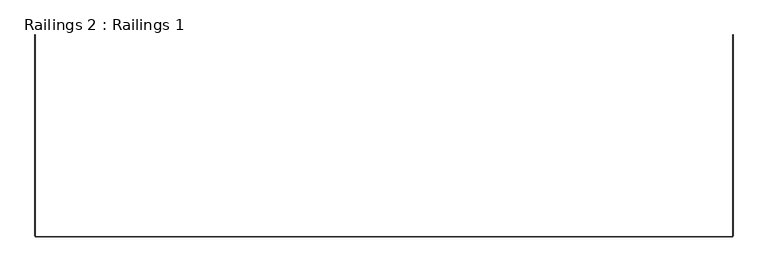
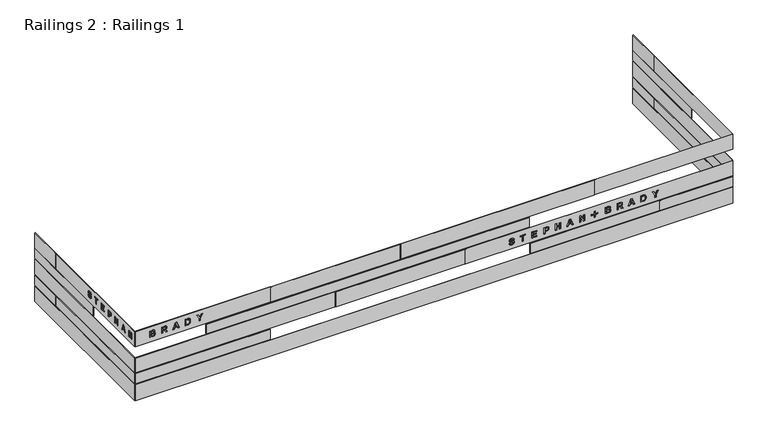
"""IFC4 building model written with IfcOpenShell, lengths in millimetres: railing geometry, Railings 2 : Railings 1."""

from ifc_helpers import new_model, si_unit, frame, origin, place, context, project, spatial, polyline, outline, extrude, source, transform, mapped, element, save


def railings_2_railings_1_346be623(model_context):
    return source(origin(), model_context, "Body", "SweptSolid", [
        extrude(outline(polyline([(-635.7738191, 4458.9611535), (-635.7738191, 4170.7510115), (-3091.5141621, 4170.7510115), (-3091.5141621, 4458.9611535), (-635.7738191, 4458.9611535)]), holes=[polyline([(-1665.1455091, 4296.7227585), (-1666.4698877, 4291.2327602), (-1668.3360732, 4286.5234788), (-1670.7440658, 4282.5949142), (-1673.6938655, 4279.4470663), (-1677.1955571, 4277.0342631), (-1681.2592258, 4275.3108322), (-1685.8848714, 4274.2767736), (-1691.072494, 4273.9320875), (-1696.5086477, 4274.2386941), (-1701.2307383, 4275.1585142), (-1705.2387656, 4276.6915475), (-1708.5327298, 4278.8377942), (-1711.7959882, 4282.2929121), (-1713.7539433, 4286.1173232), (-1714.406595, 4290.3110276), (-1713.7892085, 4294.2128728), (-1711.9370492, 4297.4868988), (-1708.5464083, 4300.2541255), (-1703.3135771, 4302.6355726), (-1701.1988373, 4303.3094256), (-1698.2227703, 4304.1647435), (-1694.3853762, 4305.2015261), (-1689.686655, 4306.4197736), (-1684.1266067, 4307.8194858), (-1678.0225, 4309.4734745), (-1672.5571346, 4311.2490498), (-1667.7305106, 4313.1462116), (-1663.5426279, 4315.1649599), (-1659.9934866, 4317.3052948), (-1657.0830867, 4319.5672161), (-1653.7434245, 4322.9544825), (-1651.0109737, 4326.5802851), (-1648.8857341, 4330.444624), (-1647.3677059, 4334.5474991), (-1646.4568889, 4338.8889105), (-1646.1532833, 4343.4688582), (-1646.4744958, 4347.9329702), (-1647.4381333, 4352.2502124), (-1649.0441959, 4356.4205848), (-1651.2926834, 4360.4440874), (-1654.1456904, 4364.1586649), (-1657.5653112, 4367.4022621), (-1661.5515457, 4370.174879), (-1666.104394, 4372.4765156), (-1670.133565, 4373.9641411), (-1674.4832299, 4375.1211831), (-1679.1533885, 4375.9476417), (-1684.144041, 4376.4435168), (-1689.4551873, 4376.6088085), (-1695.612066, 4376.4087649), (-1701.318061, 4375.8086338), (-1706.5731724, 4374.8084155), (-1711.3774, 4373.4081098), (-1715.730744, 4371.6077167), (-1719.6332044, 4369.4072363), (-1723.084781, 4366.8066685), (-1726.5506664, 4363.3570633), (-1729.4206749, 4359.5430077), (-1731.6948064, 4355.3645016), (-1733.373061, 4350.8215451), (-1734.4554386, 4345.9141382), (-1734.9419392, 4340.6422808), (-1710.964254, 4339.5739681), (-1709.5483894, 4345.1168707), (-1707.3508677, 4349.514387), (-1704.3716889, 4352.7665172), (-1701.5281294, 4354.5248978), (-1698.0524616, 4355.7808839), (-1693.9446857, 4356.5344756), (-1689.2048015, 4356.7856728), (-1684.2705786, 4356.5168558), (-1679.9025057, 4355.7104049), (-1676.100583, 4354.3663201), (-1672.8648103, 4352.4846013), (-1670.0131944, 4349.2597251), (-1669.0626557, 4345.1010026), (-1669.95338, 4341.1857107), (-1672.6255528, 4337.8787636), (-1674.9577759, 4336.3407271), (-1678.3266332, 4334.7772441), (-1682.7321248, 4333.1883144), (-1688.1742507, 4331.5739381), (-1694.6530108, 4329.9341152), (-1700.230818, 4328.5491881), (-1705.302444, 4327.1486505), (-1709.8678888, 4325.7325025), (-1713.9271525, 4324.300744), (-1717.4802351, 4322.8533751), (-1720.5271365, 4321.3903956), (-1724.4901292, 4318.9818814), (-1727.9976748, 4316.1686927), (-1731.0497732, 4312.9508296), (-1733.6464246, 4309.328292), (-1735.7192364, 4305.2782439), (-1737.1998162, 4300.7778491), (-1738.0881642, 4295.8271077), (-1738.3842801, 4290.4260196), (-1738.0300886, 4285.4065379), (-1736.9675139, 4280.5489956), (-1735.196556, 4275.8533927), (-1732.7172151, 4271.319729), (-1729.5901748, 4267.1529501), (-1725.8761189, 4263.5580014), (-1721.5750474, 4260.5348828), (-1716.6869604, 4258.0835943), (-1712.3377036, 4256.5245254), (-1707.5804848, 4255.3119163), (-1702.4153042, 4254.445767), (-1696.8421616, 4253.9260774), (-1690.8610571, 4253.7528475), (-1685.3975175, 4253.9153664), (-1680.2603487, 4254.4029232), (-1675.4495509, 4255.2155178), (-1670.965124, 4256.3531503), (-1666.8070681, 4257.8158206), (-1662.975383, 4259.6035288), (-1659.4700689, 4261.7162748), (-1656.2911257, 4264.1540587), (-1653.0428101, 4267.3199343), (-1650.1910238, 4270.8740121), (-1647.7357669, 4274.8162919), (-1645.6770393, 4279.1467737), (-1644.014841, 4283.8654576), (-1642.7491721, 4288.9723436), (-1641.8800324, 4294.4674317), (-1665.1455091, 4296.7227585)]), polyline([(-1876.840094, 4354.6490474), (-1841.5857748, 4354.6490474), (-1841.5857748, 4374.709586), (-1935.9533971, 4374.709586), (-1935.9533971, 4354.6490474), (-1900.8177792, 4354.6490474), (-1900.8177792, 4256.0081743), (-1876.840094, 4256.0081743), (-1876.840094, 4354.6490474)]), polyline([(-2055.9253864, 4374.709586), (-2143.7644311, 4374.709586), (-2143.7644311, 4354.6490474), (-2079.9030716, 4354.6490474), (-2079.9030716, 4328.297334), (-2139.3724788, 4328.297334), (-2139.3724788, 4308.2367954), (-2079.9030716, 4308.2367954), (-2079.9030716, 4276.0687129), (-2146.0197579, 4276.0687129), (-2146.0197579, 4256.0081743), (-2055.9253864, 4256.0081743), (-2055.9253864, 4374.709586)]), polyline([(-2276.947415, 4374.709586), (-2315.3565952, 4374.709586), (-2322.2116017, 4374.6600755), (-2328.2220971, 4374.5115442), (-2333.3880815, 4374.263992), (-2337.7095548, 4373.9174189), (-2341.1865169, 4373.4718249), (-2343.818968, 4372.9272101), (-2348.70578, 4371.1985628), (-2353.1782961, 4368.6852575), (-2357.2365166, 4365.3872941), (-2360.8804412, 4361.3046726), (-2363.3549206, 4357.5156865), (-2365.2795156, 4353.3086488), (-2366.6542263, 4348.6835596), (-2367.4790527, 4343.6404188), (-2367.7539949, 4338.1792265), (-2367.5065071, 4332.9300507), (-2366.7640436, 4328.1160361), (-2365.5266046, 4323.7371828), (-2363.79419, 4319.7934907), (-2360.916402, 4315.180931), (-2357.562778, 4311.2795495), (-2353.733318, 4308.089346), (-2349.6435804, 4305.5740507), (-2345.5091236, 4303.6973938), (-2341.3299478, 4302.4593752), (-2337.5961949, 4301.8470984), (-2333.2484589, 4301.3708832), (-2328.2867399, 4301.0307295), (-2322.7110379, 4300.8266372), (-2316.5213528, 4300.7586065), (-2300.9251001, 4300.7586065), (-2300.9251001, 4256.0081743), (-2276.947415, 4256.0081743), (-2276.947415, 4374.709586)]), polyline([(-2485.0051544, 4374.709586), (-2508.9828396, 4374.709586), (-2508.9828396, 4327.9412298), (-2555.8698972, 4327.9412298), (-2555.8698972, 4374.709586), (-2579.8475824, 4374.709586), (-2579.8475824, 4256.0081743), (-2555.8698972, 4256.0081743), (-2555.8698972, 4307.8806912), (-2508.9828396, 4307.8806912), (-2508.9828396, 4256.0081743), (-2485.0051544, 4256.0081743), (-2485.0051544, 4374.709586)]), polyline([(-2787.0547884, 4256.0081743), (-2776.7741333, 4282.9533947), (-2729.3844494, 4282.9533947), (-2719.5637623, 4256.0081743), (-2694.1598055, 4256.0081743), (-2740.3161076, 4374.709586), (-2765.690389, 4374.709586), (-2813.09862, 4256.0081743), (-2787.0547884, 4256.0081743)]), polyline([(-2923.2156285, 4374.709586), (-2946.4644128, 4374.709586), (-2995.0299825, 4295.3150339), (-2995.0299825, 4374.709586), (-3017.2271465, 4374.709586), (-3017.2271465, 4256.0081743), (-2993.2494614, 4256.0081743), (-2945.4127925, 4333.7631631), (-2945.4127925, 4256.0081743), (-2923.2156285, 4256.0081743), (-2923.2156285, 4374.709586)])]), frame((-11008.115848, 0.0, 0.0), z_axis=(1.0, 0.0, 0.0), x_axis=(0.0, 1.0, 0.0)), (0.0, 0.0, 1.0), 6.35),
        extrude(outline(polyline([(-11008.115848, -3091.5141621), (-11008.115848, 37.1228535), (-11001.765848, 37.1228535), (-11001.765848, -3091.5141621), (-11008.115848, -3091.5141621)])), frame((0.0, 0.0, 3133.8765531), z_axis=(0.0, 0.0, 1.0), x_axis=(1.0, 0.0, 0.0)), (0.0, 0.0, 1.0), 301.8619584),
        extrude(outline(polyline([(-11008.115848, -3091.5141621), (-11008.115848, 37.1228535), (-11001.765848, 37.1228535), (-11001.765848, -3091.5141621), (-11008.115848, -3091.5141621)])), frame((0.0, 0.0, 3664.3385115), z_axis=(0.0, 0.0, 1.0), x_axis=(1.0, 0.0, 0.0)), (0.0, 0.0, 1.0), 285.75),
        extrude(outline(polyline([(-11008.115848, -3091.5141621), (-11008.115848, -635.7738191), (-11001.765848, -635.7738191), (-11001.765848, -3091.5141621), (-11008.115848, -3091.5141621)])), frame((0.0, 0.0, 3454.7885115), z_axis=(0.0, 0.0, 1.0), x_axis=(1.0, 0.0, 0.0)), (0.0, 0.0, 1.0), 190.5),
        extrude(outline(polyline([(-11008.115848, -623.0738191), (-11008.115848, 37.1228535), (-11001.765848, 37.1228535), (-11001.765848, -623.0738191), (-11008.115848, -623.0738191)])), frame((0.0, 0.0, 4170.7510115), z_axis=(0.0, 0.0, 1.0), x_axis=(1.0, 0.0, 0.0)), (0.0, 0.0, 1.0), 288.210142),
        extrude(outline(polyline([(-11008.115848, -1802.762708), (-11008.115848, 37.1228535), (-11001.765848, 37.1228535), (-11001.765848, -1802.762708), (-11008.115848, -1802.762708)])), frame((0.0, 0.0, 3969.1385115), z_axis=(0.0, 0.0, 1.0), x_axis=(1.0, 0.0, 0.0)), (0.0, 0.0, 1.0), 182.5625),
        extrude(outline(polyline([(-11008.115848, -623.0738191), (-11008.115848, 37.1228535), (-11001.765848, 37.1228535), (-11001.765848, -623.0738191), (-11008.115848, -623.0738191)])), frame((0.0, 0.0, 3454.7885115), z_axis=(0.0, 0.0, 1.0), x_axis=(1.0, 0.0, 0.0)), (0.0, 0.0, 1.0), 190.5),
        extrude(outline(polyline([(-2300.9251001, 4320.8191451), (-2314.0026572, 4320.8191451), (-2320.4810418, 4320.9360497), (-2325.7888728, 4321.2867637), (-2329.9261502, 4321.871287), (-2332.892874, 4322.6896197), (-2337.1410863, 4325.0886865), (-2340.3599347, 4328.5449377), (-2342.3880596, 4332.8550509), (-2343.0641012, 4337.8157034), (-2342.642567, 4341.900186), (-2341.3779642, 4345.478539), (-2339.2702928, 4348.5507624), (-2336.5167704, 4351.0175261), (-2333.3146144, 4352.7795002), (-2329.6638247, 4353.8366846), (-2326.9845808, 4354.1920933), (-2323.2256641, 4354.4459567), (-2318.3870747, 4354.5982747), (-2312.4688124, 4354.6490474), (-2300.9251001, 4354.6490474), (-2300.9251001, 4320.8191451)])), frame((-11008.115848, 0.0, 0.0), z_axis=(1.0, 0.0, 0.0), x_axis=(0.0, 1.0, 0.0)), (0.0, 0.0, 1.0), 6.35),
        extrude(outline(polyline([(-2752.7389522, 4347.052157), (-2736.6920051, 4303.0139333), (-2769.0845075, 4303.0139333), (-2752.7389522, 4347.052157)])), frame((-11008.115848, 0.0, 0.0), z_axis=(1.0, 0.0, 0.0), x_axis=(0.0, 1.0, 0.0)), (0.0, 0.0, 1.0), 6.35),
        extrude(outline(polyline([(-122.0929061, -635.7738191), (-122.0929061, -3091.5141621), (-128.4429061, -3091.5141621), (-128.4429061, -635.7738191), (-122.0929061, -635.7738191)])), frame((0.0, 0.0, 4170.7510115), z_axis=(0.0, 0.0, 1.0), x_axis=(1.0, 0.0, 0.0)), (0.0, 0.0, 1.0), 288.210142),
        extrude(outline(polyline([(-122.0929061, 37.1228535), (-122.0929061, -3091.5141621), (-128.4429061, -3091.5141621), (-128.4429061, 37.1228535), (-122.0929061, 37.1228535)])), frame((0.0, 0.0, 3133.8765531), z_axis=(0.0, 0.0, 1.0), x_axis=(1.0, 0.0, 0.0)), (0.0, 0.0, 1.0), 301.8619584),
        extrude(outline(polyline([(-122.0929061, 37.1228535), (-122.0929061, -3091.5141621), (-128.4429061, -3091.5141621), (-128.4429061, 37.1228535), (-122.0929061, 37.1228535)])), frame((0.0, 0.0, 3664.3385115), z_axis=(0.0, 0.0, 1.0), x_axis=(1.0, 0.0, 0.0)), (0.0, 0.0, 1.0), 285.75),
        extrude(outline(polyline([(-122.0929061, -635.7738191), (-122.0929061, -3091.5141621), (-128.4429061, -3091.5141621), (-128.4429061, -635.7738191), (-122.0929061, -635.7738191)])), frame((0.0, 0.0, 3454.7885115), z_axis=(0.0, 0.0, 1.0), x_axis=(1.0, 0.0, 0.0)), (0.0, 0.0, 1.0), 190.5),
        extrude(outline(polyline([(-122.0929061, 37.1228535), (-122.0929061, -623.0738191), (-128.4429061, -623.0738191), (-128.4429061, 37.1228535), (-122.0929061, 37.1228535)])), frame((0.0, 0.0, 4170.7510115), z_axis=(0.0, 0.0, 1.0), x_axis=(1.0, 0.0, 0.0)), (0.0, 0.0, 1.0), 288.210142),
        extrude(outline(polyline([(-122.0929061, 37.1228535), (-122.0929061, -1802.762708), (-128.4429061, -1802.762708), (-128.4429061, 37.1228535), (-122.0929061, 37.1228535)])), frame((0.0, 0.0, 3969.1385115), z_axis=(0.0, 0.0, 1.0), x_axis=(1.0, 0.0, 0.0)), (0.0, 0.0, 1.0), 182.5625),
        extrude(outline(polyline([(-122.0929061, 37.1228535), (-122.0929061, -623.0738191), (-128.4429061, -623.0738191), (-128.4429061, 37.1228535), (-122.0929061, 37.1228535)])), frame((0.0, 0.0, 3454.7885115), z_axis=(0.0, 0.0, 1.0), x_axis=(1.0, 0.0, 0.0)), (0.0, 0.0, 1.0), 190.5),
        extrude(outline(polyline([(4279.741334, -10711.8712075), (4279.741334, -10689.6870265), (4279.7870062, -10683.8015694), (4279.9240229, -10679.1003443), (4280.152384, -10675.5833513), (4280.4720896, -10673.2505904), (4282.1457331, -10668.4016841), (4285.2192187, -10664.5455111), (4288.0189027, -10662.678952), (4291.3867462, -10661.5590165), (4295.322749, -10661.1857047), (4300.2732006, -10661.833462), (4304.4117532, -10663.776734), (4307.6373249, -10666.9445779), (4309.8488342, -10671.2660512), (4310.4624463, -10673.683628), (4310.9397002, -10677.0177281), (4311.2805958, -10681.2683514), (4311.4851332, -10686.4354981), (4311.5533123, -10692.519168), (4311.5533123, -10711.8712075), (4279.741334, -10711.8712075)])), frame((0.0, -3112.4771465, 0.0), z_axis=(0.0, 1.0, 0.0), x_axis=(0.0, 0.0, 1.0)), (0.0, 0.0, 1.0), 6.35),
        extrude(outline(polyline([(4331.2577467, -10711.8712075), (4331.2577467, -10696.1710911), (4331.2830171, -10689.8323893), (4331.3588283, -10684.8193413), (4331.4851804, -10681.1319468), (4331.6620733, -10678.770206), (4332.4579498, -10674.9612508), (4333.8737114, -10671.7371474), (4335.9093582, -10669.0978957), (4339.9836914, -10666.4577166), (4345.169923, -10665.577657), (4350.1549187, -10666.336465), (4354.1077684, -10668.6128891), (4356.8675762, -10672.3865276), (4358.2734461, -10677.6369785), (4358.4190037, -10679.5955518), (4358.5322151, -10682.6224378), (4358.6130805, -10686.7176365), (4358.6615997, -10691.8811479), (4358.6777727, -10698.112972), (4358.6777727, -10711.8712075), (4331.2577467, -10711.8712075)])), frame((0.0, -3112.4771465, 0.0), z_axis=(0.0, 1.0, 0.0), x_axis=(0.0, 0.0, 1.0)), (0.0, 0.0, 1.0), 6.35),
        extrude(outline(polyline([(4328.1715099, -10479.612046), (4328.2298591, -10473.2459039), (4328.4049066, -10467.9138735), (4328.6966524, -10463.6159551), (4329.1050965, -10460.3521485), (4329.630239, -10458.1224538), (4331.6159374, -10454.3052296), (4334.6555746, -10451.4167514), (4338.667775, -10449.5986723), (4343.5711634, -10448.992646), (4348.9915521, -10449.7904029), (4353.2564567, -10452.1836738), (4356.2652593, -10456.0310369), (4357.9173418, -10461.1910707), (4358.0942347, -10463.3723251), (4358.2205868, -10467.0079036), (4358.2963981, -10472.0978062), (4358.3216685, -10478.6420329), (4358.3216685, -10497.3041205), (4328.1715099, -10497.3041205), (4328.1715099, -10479.612046)])), frame((0.0, -3112.4771465, 0.0), z_axis=(0.0, 1.0, 0.0), x_axis=(0.0, 0.0, 1.0)), (0.0, 0.0, 1.0), 6.35),
        extrude(outline(polyline([(4350.7247782, -10259.3552553), (4306.6865544, -10275.4022023), (4306.6865544, -10243.0096999), (4350.7247782, -10259.3552553)])), frame((0.0, -3112.4771465, 0.0), z_axis=(0.0, 1.0, 0.0), x_axis=(0.0, 0.0, 1.0)), (0.0, 0.0, 1.0), 6.35),
        extrude(outline(polyline([(4279.741334, -10070.7944726), (4279.741334, -10052.9707138), (4279.8672482, -10046.9220937), (4280.2449907, -10042.1103589), (4280.8745615, -10038.5355093), (4282.0701279, -10034.8836892), (4283.7155644, -10031.6710231), (4285.810871, -10028.8975111), (4288.6301326, -10026.500402), (4292.447434, -10024.4169449), (4297.2627752, -10022.6471398), (4300.6827854, -10021.7761311), (4304.5655828, -10021.0986799), (4308.9111673, -10020.6147862), (4313.7195389, -10020.32445), (4318.9906976, -10020.2276712), (4324.2382274, -10020.32445), (4328.9742282, -10020.6147862), (4333.1987002, -10021.0986799), (4336.9116433, -10021.7761311), (4340.1130574, -10022.6471398), (4344.6628661, -10024.4751622), (4348.4934595, -10026.7332711), (4351.6048378, -10029.4214665), (4354.059752, -10032.5845706), (4355.9209531, -10036.2674056), (4357.188441, -10040.4699713), (4357.684228, -10043.5700024), (4358.0383616, -10047.8697988), (4358.2508418, -10053.3693604), (4358.3216685, -10060.0686872), (4358.3216685, -10070.7944726), (4279.741334, -10070.7944726)])), frame((0.0, -3112.4771465, 0.0), z_axis=(0.0, 1.0, 0.0), x_axis=(0.0, 0.0, 1.0)), (0.0, 0.0, 1.0), 6.35),
        extrude(outline(polyline([(4458.9611535, -8546.025505), (4458.9611535, -11001.765848), (4170.7510115, -11001.765848), (4170.7510115, -8546.025505), (4458.9611535, -8546.025505)]), holes=[polyline([(4378.3822071, -10688.4332428), (4378.33532, -10683.0880441), (4378.1946588, -10678.315728), (4377.9602236, -10674.1162946), (4377.6320142, -10670.4897439), (4377.2100306, -10667.4360759), (4376.1457365, -10662.9858034), (4374.5157559, -10658.8590746), (4372.3200889, -10655.0558896), (4369.5676999, -10651.616846), (4366.2675534, -10648.5825411), (4362.4196493, -10645.9529751), (4358.1318699, -10643.9303113), (4353.5120975, -10642.716713), (4348.5603321, -10642.3121803), (4344.4842021, -10642.5919516), (4340.5797487, -10643.4312656), (4336.8469719, -10644.8301224), (4333.2858716, -10646.7885218), (4330.0277844, -10649.225784), (4327.2040471, -10652.0612292), (4324.8146595, -10655.2948574), (4322.8596218, -10658.9266685), (4320.9996379, -10653.833694), (4318.581966, -10649.3658726), (4315.6066062, -10645.5232041), (4312.0735583, -10642.3056888), (4308.094337, -10639.7638673), (4303.7804564, -10637.9482805), (4299.1319167, -10636.8589285), (4294.1487178, -10636.4958111), (4290.1220854, -10636.7309535), (4286.1509784, -10637.4363807), (4282.2353967, -10638.6120927), (4278.3753404, -10640.2580894), (4274.7357047, -10642.311137), (4271.481385, -10644.7080013), (4268.6123811, -10647.4486825), (4266.1286932, -10650.5331804), (4264.0580839, -10653.9791728), (4262.4283158, -10657.8043374), (4261.239389, -10662.0086741), (4260.4913035, -10666.5921831), (4260.2884704, -10669.0576073), (4260.1127367, -10672.4625449), (4259.9641023, -10676.806996), (4259.8425673, -10682.0909605), (4259.7481317, -10688.3144384), (4259.6807954, -10695.4774297), (4259.6807954, -10735.8488927), (4378.3822071, -10735.8488927), (4378.3822071, -10688.4332428)]), polyline([(4378.3822071, -10521.2818057), (4378.3822071, -10470.8912017), (4378.2933098, -10464.8442045), (4378.026618, -10459.3745888), (4377.5821317, -10454.4823544), (4376.9598509, -10450.1675014), (4376.1597756, -10446.4300298), (4375.1819057, -10443.2699396), (4373.2702798, -10439.1776969), (4370.7357033, -10435.5151671), (4367.5781761, -10432.2823504), (4363.7976985, -10429.4792467), (4359.5588177, -10427.2145304), (4355.0260815, -10425.5968759), (4350.1994896, -10424.6262832), (4345.0790423, -10424.3027523), (4339.9178678, -10424.6163095), (4335.1293416, -10425.5569811), (4330.7134636, -10427.1247671), (4326.6702338, -10429.3196675), (4322.9996523, -10432.1416823), (4320.2750582, -10434.9701916), (4317.9083716, -10438.2297664), (4315.8995923, -10441.9204066), (4314.2487205, -10446.0421122), (4312.9557561, -10450.5948832), (4312.0206991, -10455.5787196), (4309.699646, -10451.8697062), (4307.2675422, -10448.4990614), (4304.7243876, -10445.4667851), (4302.0701823, -10442.7728775), (4299.5658051, -10440.6124747), (4296.3882425, -10438.1708237), (4292.5374945, -10435.4479246), (4288.0135612, -10432.4437774), (4282.8164424, -10429.158382), (4259.6807954, -10414.687938), (4259.6807954, -10443.3227988), (4285.5002072, -10460.5882901), (4290.6190572, -10464.0432431), (4294.9200544, -10467.032293), (4298.403199, -10469.5554399), (4301.0684908, -10471.6126837), (4302.9159299, -10473.2040245), (4305.9465253, -10476.7013112), (4307.8457479, -10480.401225), (4308.5866013, -10483.4296565), (4309.0311134, -10487.4466483), (4309.1792841, -10492.4522003), (4309.1792841, -10497.3041205), (4259.6807954, -10497.3041205), (4259.6807954, -10521.2818057), (4378.3822071, -10521.2818057)]), polyline([(4259.6807954, -10225.039419), (4286.6260159, -10235.3200741), (4286.6260159, -10282.709758), (4259.6807954, -10292.5304451), (4259.6807954, -10317.9344019), (4378.3822071, -10271.7780999), (4378.3822071, -10246.4038184), (4259.6807954, -10198.9955874), (4259.6807954, -10225.039419)]), polyline([(4378.3822071, -10051.0900383), (4378.2915489, -10045.4604754), (4378.0195743, -10040.3929638), (4377.5662832, -10035.8875033), (4376.9316758, -10031.9440941), (4376.115752, -10028.562736), (4374.2786622, -10023.5413997), (4371.8443559, -10018.8934395), (4368.8128331, -10014.6188557), (4365.1840939, -10010.717648), (4361.9013692, -10007.8881773), (4358.3369513, -10005.3429964), (4354.4908401, -10003.0821055), (4350.3630356, -10001.1055044), (4345.9535378, -9999.4131932), (4342.0142635, -9998.2290385), (4337.780348, -9997.2601845), (4333.2517913, -9996.5066315), (4328.4285933, -9995.9683793), (4323.3107541, -9995.645428), (4317.8982737, -9995.5377776), (4312.197861, -9995.6831126), (4306.8213547, -9996.1191178), (4301.768755, -9996.845793), (4297.0400617, -9997.8631383), (4292.6352748, -9999.1711536), (4287.65078, -10001.0990871), (4283.0614125, -10003.3307478), (4278.8671723, -10005.8661358), (4275.0680594, -10008.705251), (4271.6640739, -10011.8480935), (4268.7948382, -10015.2291131), (4266.2594502, -10019.1551854), (4264.05791, -10023.6263106), (4262.1902175, -10028.6424885), (4261.2868255, -10032.0211758), (4260.5841874, -10035.8260012), (4260.0823029, -10040.0569646), (4259.7811723, -10044.7140661), (4259.6807954, -10049.7973057), (4259.6807954, -10094.7721578), (4378.3822071, -10094.7721578), (4378.3822071, -10051.0900383)]), polyline([(4309.6392521, -9838.3457459), (4378.3822071, -9881.8498133), (4378.3822071, -9853.7695106), (4331.2855673, -9825.7448492), (4378.3822071, -9798.332242), (4378.3822071, -9770.745292), (4309.4778923, -9814.3680608), (4259.6807954, -9814.3680608), (4259.6807954, -9838.3457459), (4309.6392521, -9838.3457459)])]), frame((0.0, -3112.4771465, 0.0), z_axis=(0.0, 1.0, 0.0), x_axis=(0.0, 0.0, 1.0)), (0.0, 0.0, 1.0), 6.35),
        extrude(outline(polyline([(-128.4429061, -3112.4771465), (-2634.8810606, -3112.4771465), (-2634.8810606, -3106.1271465), (-128.4429061, -3106.1271465), (-128.4429061, -3112.4771465)])), frame((0.0, 0.0, 4170.7510115), z_axis=(0.0, 0.0, 1.0), x_axis=(1.0, 0.0, 0.0)), (0.0, 0.0, 1.0), 288.210142),
        extrude(outline(polyline([(3950.0885115, -4994.2588384), (3664.3385115, -4994.2588384), (3664.3385115, -128.4429061), (3950.0885115, -128.4429061), (3950.0885115, -4994.2588384)]), holes=[polyline([(3778.3258244, -4174.8438457), (3772.8358261, -4173.5194672), (3768.1265447, -4171.6532816), (3764.1979801, -4169.245289), (3761.0501322, -4166.2954894), (3758.637329, -4162.7937978), (3756.9138981, -4158.7301291), (3755.8798395, -4154.1044835), (3755.5351534, -4148.9168608), (3755.84176, -4143.4807071), (3756.76158, -4138.7586166), (3758.2946134, -4134.7505893), (3760.4408601, -4131.4566251), (3763.895978, -4128.1933667), (3767.7203891, -4126.2354116), (3771.9140935, -4125.5827599), (3775.8159387, -4126.2001464), (3779.0899647, -4128.0523057), (3781.8571914, -4131.4429466), (3784.2386385, -4136.6757778), (3784.9124915, -4138.7905176), (3785.7678094, -4141.7665846), (3786.804592, -4145.6039786), (3788.0228395, -4150.3026998), (3789.4225517, -4155.8627481), (3791.0765404, -4161.9668549), (3792.8521157, -4167.4322203), (3794.7492775, -4172.2588443), (3796.7680258, -4176.446727), (3798.9083607, -4179.9958683), (3801.170282, -4182.9062682), (3804.5575484, -4186.2459303), (3808.183351, -4188.9783812), (3812.0476899, -4191.1036208), (3816.150565, -4192.621649), (3820.4919764, -4193.532466), (3825.0719241, -4193.8360716), (3829.5360361, -4193.5148591), (3833.8532783, -4192.5512216), (3838.0236507, -4190.945159), (3842.0471533, -4188.6966714), (3845.7617308, -4185.8436645), (3849.005328, -4182.4240437), (3851.7779449, -4178.4378092), (3854.0795815, -4173.8849609), (3855.567207, -4169.8557899), (3856.724249, -4165.506125), (3857.5507076, -4160.8359663), (3858.0465827, -4155.8453139), (3858.2118744, -4150.5341676), (3858.0118308, -4144.3772889), (3857.4116997, -4138.6712939), (3856.4114814, -4133.4161825), (3855.0111757, -4128.6119548), (3853.2107826, -4124.2586108), (3851.0103022, -4120.3561505), (3848.4097344, -4116.9045739), (3844.9601292, -4113.4386884), (3841.1460736, -4110.56868), (3836.9675675, -4108.2945485), (3832.424611, -4106.6162939), (3827.5172041, -4105.5339163), (3822.2453467, -4105.0474157), (3821.177034, -4129.0251008), (3826.7199366, -4130.4409655), (3831.1174529, -4132.6384872), (3834.3695831, -4135.617666), (3836.1279637, -4138.4612255), (3837.3839498, -4141.9368933), (3838.1375415, -4146.0446692), (3838.3887387, -4150.7845534), (3838.1199217, -4155.7187763), (3837.3134708, -4160.0868492), (3835.969386, -4163.8887719), (3834.0876672, -4167.1245446), (3830.862791, -4169.9761605), (3826.7040685, -4170.9266992), (3822.7887766, -4170.0359749), (3819.4818295, -4167.3638021), (3817.943793, -4165.031579), (3816.38031, -4161.6627217), (3814.7913803, -4157.2572301), (3813.177004, -4151.8151042), (3811.5371811, -4145.336344), (3810.152254, -4139.7585369), (3808.7517164, -4134.6869109), (3807.3355684, -4130.121466), (3805.9038099, -4126.0622023), (3804.4564409, -4122.5091198), (3802.9934615, -4119.4622184), (3800.5849473, -4115.4992257), (3797.7717586, -4111.9916801), (3794.5538955, -4108.9395817), (3790.9313579, -4106.3429303), (3786.8813098, -4104.2701185), (3782.380915, -4102.7895386), (3777.4301736, -4101.9011907), (3772.0290854, -4101.6050748), (3767.0096038, -4101.9592663), (3762.1520615, -4103.021841), (3757.4564586, -4104.7927988), (3752.9227949, -4107.2721398), (3748.756016, -4110.3991801), (3745.1610673, -4114.113236), (3742.1379487, -4118.4143075), (3739.6866602, -4123.3023945), (3738.1275913, -4127.6516513), (3736.9149822, -4132.4088701), (3736.0488329, -4137.5740507), (3735.5291432, -4143.1471933), (3735.3559134, -4149.1282977), (3735.5184323, -4154.5918374), (3736.0059891, -4159.7290061), (3736.8185837, -4164.5398039), (3737.9562162, -4169.0242308), (3739.4188865, -4173.1822868), (3741.2065947, -4177.0139718), (3743.3193407, -4180.519286), (3745.7571246, -4183.6982292), (3748.9230002, -4186.9465448), (3752.477078, -4189.7983311), (3756.4193577, -4192.253588), (3760.7498396, -4194.3123156), (3765.4685235, -4195.9745139), (3770.5754095, -4197.2401828), (3776.0704976, -4198.1093224), (3778.3258244, -4174.8438457)]), polyline([(3836.2521133, -3963.1492608), (3836.2521133, -3998.4035801), (3856.3126519, -3998.4035801), (3856.3126519, -3904.0359578), (3836.2521133, -3904.0359578), (3836.2521133, -3939.1715757), (3737.6112402, -3939.1715757), (3737.6112402, -3963.1492608), (3836.2521133, -3963.1492608)]), polyline([(3856.3126519, -3784.0639684), (3856.3126519, -3696.2249238), (3836.2521133, -3696.2249238), (3836.2521133, -3760.0862833), (3809.9003999, -3760.0862833), (3809.9003999, -3700.616876), (3789.8398613, -3700.616876), (3789.8398613, -3760.0862833), (3757.6717788, -3760.0862833), (3757.6717788, -3693.969597), (3737.6112402, -3693.969597), (3737.6112402, -3784.0639684), (3856.3126519, -3784.0639684)]), polyline([(3856.3126519, -3563.0419399), (3856.3126519, -3524.6327597), (3856.2631414, -3517.7777532), (3856.1146101, -3511.7672577), (3855.8670579, -3506.6012734), (3855.5204848, -3502.2798001), (3855.0748908, -3498.8028379), (3854.530276, -3496.1703868), (3852.8016287, -3491.2835749), (3850.2883234, -3486.8110587), (3846.99036, -3482.7528383), (3842.9077385, -3479.1089136), (3839.1187524, -3476.6344343), (3834.9117147, -3474.7098393), (3830.2866255, -3473.3351286), (3825.2434847, -3472.5103022), (3819.7822924, -3472.23536), (3814.5331166, -3472.4828478), (3809.719102, -3473.2253112), (3805.3402487, -3474.4627503), (3801.3965566, -3476.1951649), (3796.7839969, -3479.0729529), (3792.8826154, -3482.4265769), (3789.6924119, -3486.2560369), (3787.1771166, -3490.3457745), (3785.3004597, -3494.4802312), (3784.0624411, -3498.6594071), (3783.4501643, -3502.39316), (3782.9739491, -3506.7408959), (3782.6337954, -3511.7026149), (3782.4297031, -3517.278317), (3782.3616724, -3523.4680021), (3782.3616724, -3539.0642548), (3737.6112402, -3539.0642548), (3737.6112402, -3563.0419399), (3856.3126519, -3563.0419399)]), polyline([(3856.3126519, -3354.9842004), (3856.3126519, -3331.0065153), (3809.5442957, -3331.0065153), (3809.5442957, -3284.1194577), (3856.3126519, -3284.1194577), (3856.3126519, -3260.1417725), (3737.6112402, -3260.1417725), (3737.6112402, -3284.1194577), (3789.4837571, -3284.1194577), (3789.4837571, -3331.0065153), (3737.6112402, -3331.0065153), (3737.6112402, -3354.9842004), (3856.3126519, -3354.9842004)]), polyline([(3737.6112402, -3052.9345665), (3764.5564606, -3063.2152216), (3764.5564606, -3110.6049054), (3737.6112402, -3120.4255925), (3737.6112402, -3145.8295494), (3856.3126519, -3099.6732473), (3856.3126519, -3074.2989659), (3737.6112402, -3026.8907349), (3737.6112402, -3052.9345665)]), polyline([(3856.3126519, -2916.7737264), (3856.3126519, -2893.5249421), (3776.9180998, -2844.9593723), (3856.3126519, -2844.9593723), (3856.3126519, -2822.7622084), (3737.6112402, -2822.7622084), (3737.6112402, -2846.7398935), (3815.366229, -2894.5765624), (3737.6112402, -2894.5765624), (3737.6112402, -2916.7737264), (3856.3126519, -2916.7737264)]), polyline([(3856.3126519, -2398.8843557), (3856.2657648, -2393.5391569), (3856.1251036, -2388.7668409), (3855.8906683, -2384.5674075), (3855.5624589, -2380.9408568), (3855.1404754, -2377.8871888), (3854.0761812, -2373.4369163), (3852.4462007, -2369.3101875), (3850.2505337, -2365.5070025), (3847.4981447, -2362.0679588), (3844.1979981, -2359.033654), (3840.350094, -2356.404088), (3836.0623147, -2354.3814242), (3831.4425423, -2353.1678259), (3826.4907769, -2352.7632931), (3822.4146469, -2353.0430645), (3818.5101935, -2353.8823785), (3814.7774166, -2355.2812352), (3811.2163163, -2357.2396347), (3807.9582292, -2359.6768969), (3805.1344918, -2362.5123421), (3802.7451043, -2365.7459702), (3800.7900665, -2369.3777813), (3798.9300827, -2364.2848069), (3796.5124108, -2359.8169854), (3793.5370509, -2355.974317), (3790.0040031, -2352.7568017), (3786.0247817, -2350.2149802), (3781.7109012, -2348.3993934), (3777.0623615, -2347.3100413), (3772.0791626, -2346.946924), (3768.0525302, -2347.1820664), (3764.0814232, -2347.8874935), (3760.1658415, -2349.0632055), (3756.3057852, -2350.7092023), (3752.6661495, -2352.7622499), (3749.4118298, -2355.1591142), (3746.5428259, -2357.8997953), (3744.059138, -2360.9842932), (3741.9885286, -2364.4302856), (3740.3587606, -2368.2554502), (3739.1698338, -2372.459787), (3738.4217483, -2377.0432959), (3738.2189152, -2379.5087201), (3738.0431814, -2382.9136578), (3737.8945471, -2387.2581088), (3737.7730121, -2392.5420733), (3737.6785765, -2398.7655512), (3737.6112402, -2405.9285426), (3737.6112402, -2446.3000055), (3856.3126519, -2446.3000055), (3856.3126519, -2398.8843557)]), polyline([(3856.3126519, -2231.7329185), (3856.3126519, -2181.3423146), (3856.2237546, -2175.2953174), (3855.9570628, -2169.8257017), (3855.5125765, -2164.9334673), (3854.8902957, -2160.6186143), (3854.0902204, -2156.8811427), (3853.1123505, -2153.7210525), (3851.2007246, -2149.6288097), (3848.666148, -2145.96628), (3845.5086209, -2142.7334633), (3841.7281432, -2139.9303596), (3837.4892625, -2137.6656433), (3832.9565262, -2136.0479888), (3828.1299344, -2135.0773961), (3823.009487, -2134.7538652), (3817.8483126, -2135.0674224), (3813.0597863, -2136.008094), (3808.6439084, -2137.57588), (3804.6006786, -2139.7707804), (3800.9300971, -2142.5927951), (3798.205503, -2145.4213045), (3795.8388163, -2148.6808793), (3793.8300371, -2152.3715194), (3792.1791653, -2156.493225), (3790.8862009, -2161.045996), (3789.9511439, -2166.0298325), (3787.6300908, -2162.3208191), (3785.197987, -2158.9501742), (3782.6548324, -2155.917898), (3780.0006271, -2153.2239903), (3777.4962499, -2151.0635875), (3774.3186873, -2148.6219366), (3770.4679393, -2145.8990375), (3765.944006, -2142.8948902), (3760.7468872, -2139.6094948), (3737.6112402, -2125.1390509), (3737.6112402, -2153.7739117), (3763.4306519, -2171.039403), (3768.5495019, -2174.4943559), (3772.8504992, -2177.4834059), (3776.3336438, -2180.0065527), (3778.9989356, -2182.0637966), (3780.8463747, -2183.6551374), (3783.8769701, -2187.1524241), (3785.7761927, -2190.8523378), (3786.5170461, -2193.8807694), (3786.9615582, -2197.8977612), (3787.1097289, -2202.9033132), (3787.1097289, -2207.7552334), (3737.6112402, -2207.7552334), (3737.6112402, -2231.7329185), (3856.3126519, -2231.7329185)]), polyline([(3737.6112402, -1935.4905319), (3764.5564606, -1945.771187), (3764.5564606, -1993.1608709), (3737.6112402, -2002.981558), (3737.6112402, -2028.3855148), (3856.3126519, -1982.2292127), (3856.3126519, -1956.8549313), (3737.6112402, -1909.4467003), (3737.6112402, -1935.4905319)]), polyline([(3856.3126519, -1761.5411511), (3856.2219936, -1755.9115883), (3855.950019, -1750.8440767), (3855.496728, -1746.3386162), (3854.8621206, -1742.3952069), (3854.0461968, -1739.0138488), (3852.209107, -1733.9925125), (3849.7748007, -1729.3445524), (3846.7432779, -1725.0699685), (3843.1145386, -1721.1687608), (3839.831814, -1718.3392901), (3836.2673961, -1715.7941093), (3832.4212849, -1713.5332183), (3828.2934804, -1711.5566173), (3823.8839826, -1709.8643061), (3819.9447083, -1708.6801513), (3815.7107928, -1707.7112974), (3811.182236, -1706.9577444), (3806.3590381, -1706.4194922), (3801.2411989, -1706.0965409), (3795.8287185, -1705.9888905), (3790.1283058, -1706.1342255), (3784.7517995, -1706.5702306), (3779.6991997, -1707.2969058), (3774.9705064, -1708.3142511), (3770.5657196, -1709.6222665), (3765.5812248, -1711.5502), (3760.9918572, -1713.7818607), (3756.7976171, -1716.3172487), (3752.9985042, -1719.1563639), (3749.5945186, -1722.2992063), (3746.725283, -1725.6802259), (3744.189895, -1729.6062983), (3741.9883547, -1734.0774234), (3740.1206622, -1739.0936014), (3739.2172703, -1742.4722887), (3738.5146321, -1746.277114), (3738.0127477, -1750.5080775), (3737.7116171, -1755.165179), (3737.6112402, -1760.2484186), (3737.6112402, -1805.2232706), (3856.3126519, -1805.2232706), (3856.3126519, -1761.5411511)]), polyline([(3787.5696968, -1548.7968588), (3856.3126519, -1592.3009262), (3856.3126519, -1564.2206235), (3809.2160121, -1536.1959621), (3856.3126519, -1508.7833548), (3856.3126519, -1481.1964049), (3787.4083371, -1524.8191736), (3737.6112402, -1524.8191736), (3737.6112402, -1548.7968588), (3787.5696968, -1548.7968588)]), polyline([(3785.863364, -2652.3296426), (3785.863364, -2700.5817664), (3808.060528, -2700.5817664), (3808.060528, -2652.3296426), (3856.3126519, -2652.3296426), (3856.3126519, -2630.1324786), (3808.060528, -2630.1324786), (3808.060528, -2581.8803548), (3785.863364, -2581.8803548), (3785.863364, -2630.1324786), (3737.6112402, -2630.1324786), (3737.6112402, -2652.3296426), (3785.863364, -2652.3296426)])]), frame((0.0, -3112.4771465, 0.0), z_axis=(0.0, 1.0, 0.0), x_axis=(0.0, 0.0, 1.0)), (0.0, 0.0, 1.0), 6.35),
        extrude(outline(polyline([(-128.4429061, -3112.4771465), (-1455.1921717, -3112.4771465), (-1455.1921717, -3106.1271465), (-128.4429061, -3106.1271465), (-128.4429061, -3112.4771465)])), frame((0.0, 0.0, 3454.7885115), z_axis=(0.0, 0.0, 1.0), x_axis=(1.0, 0.0, 0.0)), (0.0, 0.0, 1.0), 190.5),
        extrude(outline(polyline([(-128.4429061, -3112.4771465), (-11001.765848, -3112.4771465), (-11001.765848, -3106.1271465), (-128.4429061, -3106.1271465), (-128.4429061, -3112.4771465)])), frame((0.0, 0.0, 3133.8765531), z_axis=(0.0, 0.0, 1.0), x_axis=(1.0, 0.0, 0.0)), (0.0, 0.0, 1.0), 301.8619584),
        extrude(outline(polyline([(3802.422211, -3539.0642548), (3802.422211, -3525.9866977), (3802.5391156, -3519.5083131), (3802.8898296, -3514.2004821), (3803.4743529, -3510.0632047), (3804.2926855, -3507.0964808), (3806.6917524, -3502.8482686), (3810.1480036, -3499.6294202), (3814.4581168, -3497.6012953), (3819.4187693, -3496.9252536), (3823.5032519, -3497.3467879), (3827.0816049, -3498.6113907), (3830.1538283, -3500.719062), (3832.620592, -3503.4725845), (3834.382566, -3506.6747405), (3835.4397505, -3510.3255302), (3835.7951592, -3513.0047741), (3836.0490226, -3516.7636907), (3836.2013406, -3521.6022802), (3836.2521133, -3527.5205425), (3836.2521133, -3539.0642548), (3802.422211, -3539.0642548)])), frame((0.0, -3112.4771465, 0.0), z_axis=(0.0, 1.0, 0.0), x_axis=(0.0, 0.0, 1.0)), (0.0, 0.0, 1.0), 6.35),
        extrude(outline(polyline([(3828.6552229, -3087.2504027), (3784.6169992, -3103.2973498), (3784.6169992, -3070.9048474), (3828.6552229, -3087.2504027)])), frame((0.0, -3112.4771465, 0.0), z_axis=(0.0, 1.0, 0.0), x_axis=(0.0, 0.0, 1.0)), (0.0, 0.0, 1.0), 6.35),
        extrude(outline(polyline([(3757.6717788, -2422.3223204), (3757.6717788, -2400.1381394), (3757.717451, -2394.2526823), (3757.8544677, -2389.5514572), (3758.0828288, -2386.0344642), (3758.4025343, -2383.7017033), (3760.0761779, -2378.852797), (3763.1496634, -2374.996624), (3765.9493475, -2373.1300649), (3769.317191, -2372.0101294), (3773.2531938, -2371.6368176), (3778.2036454, -2372.2845749), (3782.3421979, -2374.2278468), (3785.5677697, -2377.3956908), (3787.779279, -2381.717164), (3788.3928911, -2384.1347408), (3788.870145, -2387.4688409), (3789.2110406, -2391.7194643), (3789.415578, -2396.8866109), (3789.4837571, -2402.9702808), (3789.4837571, -2422.3223204), (3757.6717788, -2422.3223204)])), frame((0.0, -3112.4771465, 0.0), z_axis=(0.0, 1.0, 0.0), x_axis=(0.0, 0.0, 1.0)), (0.0, 0.0, 1.0), 6.35),
        extrude(outline(polyline([(3809.1881914, -2422.3223204), (3809.1881914, -2406.622204), (3809.2134618, -2400.2835022), (3809.2892731, -2395.2704541), (3809.4156252, -2391.5830597), (3809.5925181, -2389.2213189), (3810.3883946, -2385.4123637), (3811.8041562, -2382.1882603), (3813.839803, -2379.5490086), (3817.9141362, -2376.9088295), (3823.1003678, -2376.0287698), (3828.0853634, -2376.7875779), (3832.0382132, -2379.064002), (3834.798021, -2382.8376404), (3836.2038908, -2388.0880914), (3836.3494484, -2390.0466647), (3836.4626599, -2393.0735507), (3836.5435252, -2397.1687494), (3836.5920444, -2402.3322608), (3836.6082175, -2408.5640849), (3836.6082175, -2422.3223204), (3809.1881914, -2422.3223204)])), frame((0.0, -3112.4771465, 0.0), z_axis=(0.0, 1.0, 0.0), x_axis=(0.0, 0.0, 1.0)), (0.0, 0.0, 1.0), 6.35),
        extrude(outline(polyline([(3806.1019547, -2190.0631589), (3806.1603039, -2183.6970167), (3806.3353514, -2178.3649864), (3806.6270972, -2174.067068), (3807.0355413, -2170.8032614), (3807.5606838, -2168.5735666), (3809.5463822, -2164.7563425), (3812.5860193, -2161.8678642), (3816.5982198, -2160.0497852), (3821.5016082, -2159.4437588), (3826.9219969, -2160.2415158), (3831.1869015, -2162.6347866), (3834.1957041, -2166.4821498), (3835.8477866, -2171.6421836), (3836.0246795, -2173.8234379), (3836.1510316, -2177.4590164), (3836.2268429, -2182.5489191), (3836.2521133, -2189.0931458), (3836.2521133, -2207.7552334), (3806.1019547, -2207.7552334), (3806.1019547, -2190.0631589)])), frame((0.0, -3112.4771465, 0.0), z_axis=(0.0, 1.0, 0.0), x_axis=(0.0, 0.0, 1.0)), (0.0, 0.0, 1.0), 6.35),
        extrude(outline(polyline([(3828.6552229, -1969.8063681), (3784.6169992, -1985.8533152), (3784.6169992, -1953.4608128), (3828.6552229, -1969.8063681)])), frame((0.0, -3112.4771465, 0.0), z_axis=(0.0, 1.0, 0.0), x_axis=(0.0, 0.0, 1.0)), (0.0, 0.0, 1.0), 6.35),
        extrude(outline(polyline([(3757.6717788, -1781.2455855), (3757.6717788, -1763.4218266), (3757.7976929, -1757.3732066), (3758.1754354, -1752.5614718), (3758.8050063, -1748.9866221), (3760.0005727, -1745.3348021), (3761.6460092, -1742.122136), (3763.7413158, -1739.3486239), (3766.5605774, -1736.9515149), (3770.3778787, -1734.8680578), (3775.19322, -1733.0982527), (3778.6132302, -1732.227244), (3782.4960275, -1731.5497928), (3786.841612, -1731.0658991), (3791.6499837, -1730.7755628), (3796.9211424, -1730.6787841), (3802.1686722, -1730.7755628), (3806.904673, -1731.0658991), (3811.129145, -1731.5497928), (3814.842088, -1732.227244), (3818.0435022, -1733.0982527), (3822.5933108, -1734.9262751), (3826.4239043, -1737.1843839), (3829.5352826, -1739.8725794), (3831.9901968, -1743.0356835), (3833.8513978, -1746.7185184), (3835.1188857, -1750.9210842), (3835.6146728, -1754.0211153), (3835.9688064, -1758.3209117), (3836.1812866, -1763.8204733), (3836.2521133, -1770.5198001), (3836.2521133, -1781.2455855), (3757.6717788, -1781.2455855)])), frame((0.0, -3112.4771465, 0.0), z_axis=(0.0, 1.0, 0.0), x_axis=(0.0, 0.0, 1.0)), (0.0, 0.0, 1.0), 6.35),
        extrude(outline(polyline([(-7366.3366161, -3112.4771465), (-11001.765848, -3112.4771465), (-11001.765848, -3106.1271465), (-7366.3366161, -3106.1271465), (-7366.3366161, -3112.4771465)])), frame((0.0, 0.0, 3664.3385115), z_axis=(0.0, 0.0, 1.0), x_axis=(1.0, 0.0, 0.0)), (0.0, 0.0, 1.0), 285.75),
        extrude(outline(polyline([(-8546.025505, -3112.4771465), (-11001.765848, -3112.4771465), (-11001.765848, -3106.1271465), (-8546.025505, -3106.1271465), (-8546.025505, -3112.4771465)])), frame((0.0, 0.0, 3454.7885115), z_axis=(0.0, 0.0, 1.0), x_axis=(1.0, 0.0, 0.0)), (0.0, 0.0, 1.0), 190.5),
        extrude(outline(polyline([(-6186.6477273, -3112.4771465), (-8533.325505, -3112.4771465), (-8533.325505, -3106.1271465), (-6186.6477273, -3106.1271465), (-6186.6477273, -3112.4771465)])), frame((0.0, 0.0, 4170.7510115), z_axis=(0.0, 0.0, 1.0), x_axis=(1.0, 0.0, 0.0)), (0.0, 0.0, 1.0), 288.210142),
        extrude(outline(polyline([(-2647.5810606, -3112.4771465), (-6173.9477273, -3112.4771465), (-6173.9477273, -3106.1271465), (-2647.5810606, -3106.1271465), (-2647.5810606, -3112.4771465)])), frame((0.0, 0.0, 4170.7510115), z_axis=(0.0, 0.0, 1.0), x_axis=(1.0, 0.0, 0.0)), (0.0, 0.0, 1.0), 288.210142),
        extrude(outline(polyline([(-5006.9588384, -3112.4771465), (-7353.6366161, -3112.4771465), (-7353.6366161, -3106.1271465), (-5006.9588384, -3106.1271465), (-5006.9588384, -3112.4771465)])), frame((0.0, 0.0, 3664.3385115), z_axis=(0.0, 0.0, 1.0), x_axis=(1.0, 0.0, 0.0)), (0.0, 0.0, 1.0), 285.75),
        extrude(outline(polyline([(-3827.2699495, -3112.4771465), (-9713.0143939, -3112.4771465), (-9713.0143939, -3106.1271465), (-3827.2699495, -3106.1271465), (-3827.2699495, -3112.4771465)])), frame((0.0, 0.0, 3969.1385115), z_axis=(0.0, 0.0, 1.0), x_axis=(1.0, 0.0, 0.0)), (0.0, 0.0, 1.0), 182.5625),
        extrude(outline(polyline([(-1467.8921717, -3112.4771465), (-3814.5699495, -3112.4771465), (-3814.5699495, -3106.1271465), (-1467.8921717, -3106.1271465), (-1467.8921717, -3112.4771465)])), frame((0.0, 0.0, 3454.7885115), z_axis=(0.0, 0.0, 1.0), x_axis=(1.0, 0.0, 0.0)), (0.0, 0.0, 1.0), 190.5),
    ])


if __name__ == "__main__":
    model = new_model("IFC4")
    model_context = context("Model", 3, world=origin())
    ifc_project = project(units=[si_unit("LENGTHUNIT", "METRE", prefix="MILLI")], contexts=[model_context])
    site = spatial("IfcSite", under=ifc_project)
    building = spatial("IfcBuilding", under=site)
    placement = place(None, origin())
    railings_2_railings_1_shape = railings_2_railings_1_346be623(model_context)
    element("IfcRailing", 1, ObjectType="Railings 2 : Railings 1", at=placement, inside=building, context=model_context, shape_type="MappedRepresentation", body=[
        mapped(railings_2_railings_1_shape, transform((0.0, 0.0, 0.0), x_axis=(1.0, 0.0, 0.0), y_axis=(0.0, 1.0, 0.0), z_axis=(0.0, 0.0, 1.0))),
    ])
    save(model, "model.ifc")

# Revit data of these elements
# Element 1 (IfcRailing, "Railings 2 : Railings 1")
#   Materials on its faces: "RAILING STEEL"
# Materials
#   "RAILING STEEL": class "Metal", colour RGB 16 16 15, transparency 0, Description = "Structural steel, ASTM A36 Grade B, mill finish", Cost = 0
